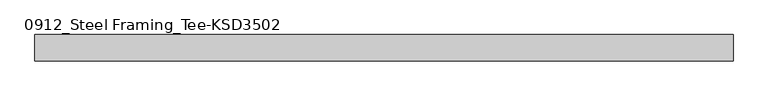
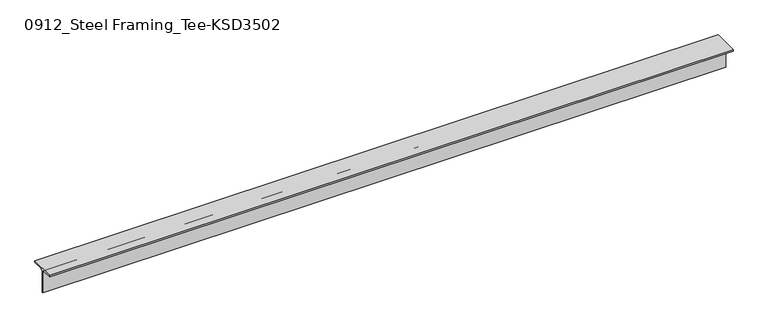
"""IFC4 building model written with IfcOpenShell, lengths in millimetres: member geometry, 0912_Steel Framing_Tee-KSD3502 : H_SB_ASB_CT-150x150x6.5x9."""

from ifc_helpers import new_model, si_unit, point, frame, frame_2d, origin, place, context, project, spatial, polyline, circle_curve, trimmed, segment, composite_curve, outline, extrude, source, transform, mapped, element, save


def member_0912_steel_framing_tee_ksd3502_f8e7eef6(model_context):
    return source(origin(), model_context, "Body", "SweptSolid", [
        extrude(outline(composite_curve([segment(polyline([(-75.0, 75.0), (75.0, 75.0), (75.0, 66.0), (16.25, 66.0)]), True, "CONTINUOUS"), segment(trimmed(circle_curve(frame_2d((16.25, 53.0)), 13.0), [point((16.25, 66.0))], [point((3.25, 53.0))], True, "CARTESIAN"), True, "CONTINUOUS"), segment(polyline([(3.25, 53.0), (3.25, -75.0), (-3.25, -75.0), (-3.25, 53.0)]), True, "CONTINUOUS"), segment(trimmed(circle_curve(frame_2d((-16.25, 53.0)), 13.0), [point((-3.25, 53.0))], [point((-16.25, 66.0))], True, "CARTESIAN"), True, "CONTINUOUS"), segment(polyline([(-16.25, 66.0), (-75.0, 66.0), (-75.0, 75.0)]), True, "CONTINUOUS")], self_intersect=False)), frame((-1965.45, 0.0, 0.0), z_axis=(1.0, 0.0, 0.0), x_axis=(0.0, 1.0, 0.0)), (0.0, 0.0, 1.0), 3968.5),
    ])


if __name__ == "__main__":
    model = new_model("IFC4")
    model_context = context("Model", 3, world=origin())
    ifc_project = project(units=[si_unit("LENGTHUNIT", "METRE", prefix="MILLI")], contexts=[model_context])
    site = spatial("IfcSite", under=ifc_project)
    building = spatial("IfcBuilding", under=site)
    placement = place(None, origin())
    member_0912_steel_framing_tee_ksd3502_shape = member_0912_steel_framing_tee_ksd3502_f8e7eef6(model_context)
    element("IfcMember", 1, ObjectType="0912_Steel Framing_Tee-KSD3502 : H_SB_ASB_CT-150x150x6.5x9", at=placement, inside=building, context=model_context, shape_type="MappedRepresentation", body=[
        mapped(member_0912_steel_framing_tee_ksd3502_shape, transform((0.0, 0.0, 0.0), x_axis=(1.0, 0.0, 0.0), y_axis=(0.0, 1.0, 0.0), z_axis=(0.0, 0.0, 1.0))),
    ])
    save(model, "model.ifc")

# Revit data of these elements
# Type "0912_Steel Framing_Tee-KSD3502 : H_SB_ASB_CT-150x150x6.5x9"
#   H_WM Code_1 = "S01AA003-00001 | Main Steel Structure Fabrication Work | Shelter/Building | Light Steel - Standard (30KG/M>Weight) | Material: (   )"
#   H_WM Code_2 = "S03AA029-00001 | Main Steel Structure Erection Work | Shelter/Building | Light Steel (30KG/M>Weight) | Material: (   )"
#   H_WM Code_3 = "S01AA010-00001 | Main Steel Structure Fabrication Work | Shelter/Building | Steel Painting/Coating | for Non-Fireproofed Steel Surface, Surface Preparation, Primer, Second & Final Coat | Material: (   )"
#   H_Q'ty Cal Type Tag = "SB-Q2"
#   Width = 15.0 cm
#   Web Thickness = 0.65 cm
#   Web Fillet = 1.3 cm
#   Section Area = 23.39 cm²
#   Perimeter = 0.60 m²/m
#   Nominal Weight = 18.40 kgf/m
#   Height = 15.0 cm
#   Flange Thickness = 0.9 cm
#   Centroid Vertical = 7.5 cm
#   Centroid Horizontal = 7.5 cm
#   Length [instance default] = 1.5000 m
#   Structural Material [instance default] = Steel, 45-345
#   Warping Constant = (empty or 0)
#   Torsional Moment of Inertia = 0
#   Section Name Key = ""
#   Plastic Modulus weak axis = 0
#   Plastic Modulus strong axis = 0
#   Moment of Inertia weak axis = 0
#   Moment of Inertia strong axis = 0
#   Elastic Modulus weak axis = 0
#   Elastic Modulus strong axis = 0
#   Bolt Spacing = 0
#   Assembly Code = ""
# Element 1 (IfcMember, "0912_Steel Framing_Tee-KSD3502 : H_SB_ASB_CT-150x150x6.5x9")
#   Structural Material = none
# Materials
#   "Steel, 45-345": class "Metal", colour RGB 189 187 185, transparency 0, Description = "Steel 345 MPa", Cost = 0
